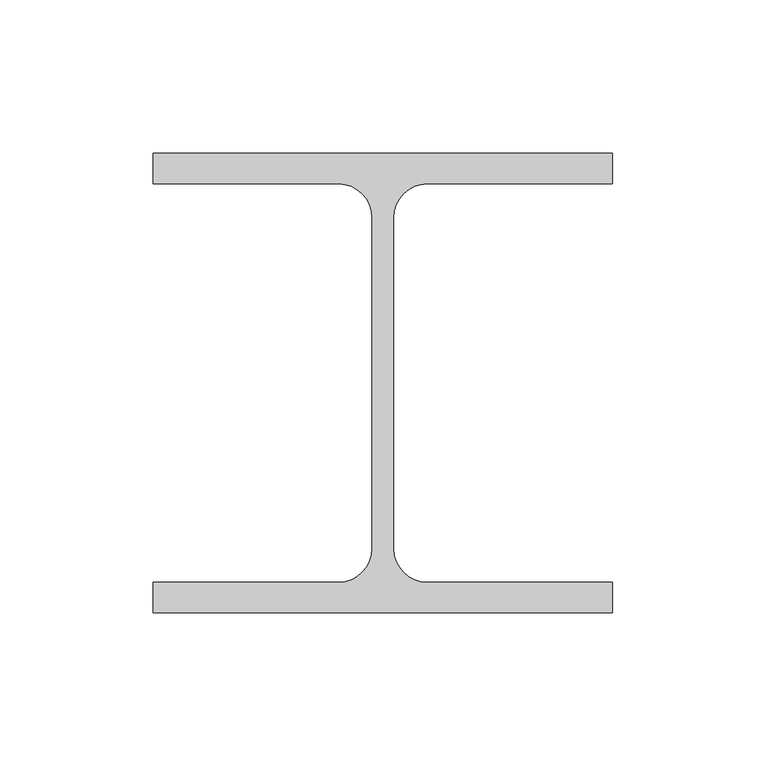
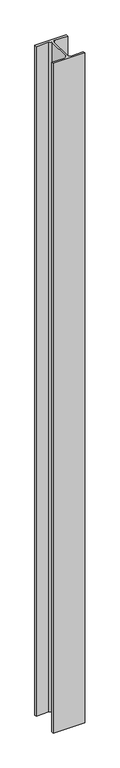
"""IFC4 building model written with IfcOpenShell, lengths in millimetres: column geometry, 0912_Steel Column_H_KSD3502 : H_SC_ASC_H-150x150x7x10."""

from ifc_helpers import new_model, si_unit, point, frame, frame_2d, origin, place, context, project, spatial, polyline, circle_curve, trimmed, segment, composite_curve, outline, extrude, source, transform, mapped, element, save


def column_781554eb(model_context):
    return source(origin(), model_context, "Body", "SweptSolid", [
        extrude(outline(composite_curve([segment(polyline([(75.0, 75.0), (75.0, 65.0), (14.5, 65.0)]), True, "CONTINUOUS"), segment(trimmed(circle_curve(frame_2d((14.5, 54.0)), 11.0), [point((14.5, 65.0))], [point((3.5, 54.0))], True, "CARTESIAN"), True, "CONTINUOUS"), segment(polyline([(3.5, 54.0), (3.5, -54.0)]), True, "CONTINUOUS"), segment(trimmed(circle_curve(frame_2d((14.5, -54.0)), 11.0), [point((3.5, -54.0))], [point((14.5, -65.0))], True, "CARTESIAN"), True, "CONTINUOUS"), segment(polyline([(14.5, -65.0), (75.0, -65.0), (75.0, -75.0), (-75.0, -75.0), (-75.0, -65.0), (-14.5, -65.0)]), True, "CONTINUOUS"), segment(trimmed(circle_curve(frame_2d((-14.5, -54.0)), 11.0), [point((-14.5, -65.0))], [point((-3.5, -54.0))], True, "CARTESIAN"), True, "CONTINUOUS"), segment(polyline([(-3.5, -54.0), (-3.5, 54.0)]), True, "CONTINUOUS"), segment(trimmed(circle_curve(frame_2d((-14.5, 54.0)), 11.0), [point((-3.5, 54.0))], [point((-14.5, 65.0))], True, "CARTESIAN"), True, "CONTINUOUS"), segment(polyline([(-14.5, 65.0), (-75.0, 65.0), (-75.0, 75.0), (75.0, 75.0)]), True, "CONTINUOUS")], self_intersect=False)), frame((0.0, 0.0, 599.9720055), z_axis=(0.0, 0.0, 1.0), x_axis=(1.0, 0.0, 0.0)), (0.0, 0.0, 1.0), 3368.0),
    ])


if __name__ == "__main__":
    model = new_model("IFC4")
    model_context = context("Model", 3, world=origin())
    ifc_project = project(units=[si_unit("LENGTHUNIT", "METRE", prefix="MILLI")], contexts=[model_context])
    site = spatial("IfcSite", under=ifc_project)
    building = spatial("IfcBuilding", under=site)
    placement = place(None, origin())
    column_shape = column_781554eb(model_context)
    element("IfcColumn", 1, ObjectType="0912_Steel Column_H_KSD3502 : H_SC_ASC_H-150x150x7x10", at=placement, inside=building, context=model_context, shape_type="MappedRepresentation", body=[
        mapped(column_shape, transform((0.0, 0.0, 0.0), x_axis=(1.0, 0.0, 0.0), y_axis=(0.0, 1.0, 0.0), z_axis=(0.0, 0.0, 1.0))),
    ])
    save(model, "model.ifc")

# Revit data of these elements
# Type "0912_Steel Column_H_KSD3502 : H_SC_ASC_H-150x150x7x10"
#   H_WM Code_1 = "S01AA002-00001 | Main Steel Structure Fabrication Work | Shelter/Building | Medium Steel - Standard (90KG/M>Weight≥30KG/M) | Material: (   )"
#   H_WM Code_2 = "S03AA028-00001 | Main Steel Structure Erection Work | Shelter/Building | Medium Steel (90KG/M>Weight≥30KG/M) | Material: (   )"
#   H_WM Code_3 = "S01AA010-00001 | Main Steel Structure Fabrication Work | Shelter/Building | Steel Painting/Coating | for Non-Fireproofed Steel Surface, Surface Preparation, Primer, Second & Final Coat | Material: (   )"
#   H_Q'ty Cal Type Tag = "SC-Q2"
#   Width = 15.0 cm
#   Web Thickness = 0.7 cm
#   Web Fillet = 1.1 cm
#   Warping Constant = 27562.5 cm⁶
#   Torsional Moment of Inertia = 11.6007 cm⁴
#   Section Area = 40.14 cm²
#   Plastic Modulus weak axis = 115.0 cm³
#   Plastic Modulus strong axis = 246.0 cm³
#   Perimeter = 0.87 m²/m
#   Nominal Weight = 31.50 kgf/m
#   Moment of Inertia weak axis = 563.00 cm⁴
#   Moment of Inertia strong axis = 1640.00 cm⁴
#   Height = 15.0 cm
#   Flange Thickness = 1.0 cm
#   Elastic Modulus weak axis = 75.1 cm³
#   Elastic Modulus strong axis = 219.0 cm³
#   Centroid Vertical = 7.5 cm
#   Centroid Horizontal = 7.5 cm
#   Structural Material [instance default] = Steel, 45-345
#   Section Name Key = ""
#   Bolt Spacing = 0
#   Assembly Code = ""
# Element 1 (IfcColumn, "0912_Steel Column_H_KSD3502 : H_SC_ASC_H-150x150x7x10")
#   Structural Material = A03AD029-00005_Anchor Bolt (Installation only)_M24
#   Materials on its faces: "A03AD029-00005_Anchor Bolt (Installation only)_M24"
# Materials
#   "Steel, 45-345": class "Metal", colour RGB 189 187 185, transparency 0, Description = "Steel 345 MPa", Cost = 0
#   "A03AD029-00005_Anchor Bolt (Installation only)_M24": class "Unassigned", colour RGB 84 83 81, transparency 0, Cost = 0
